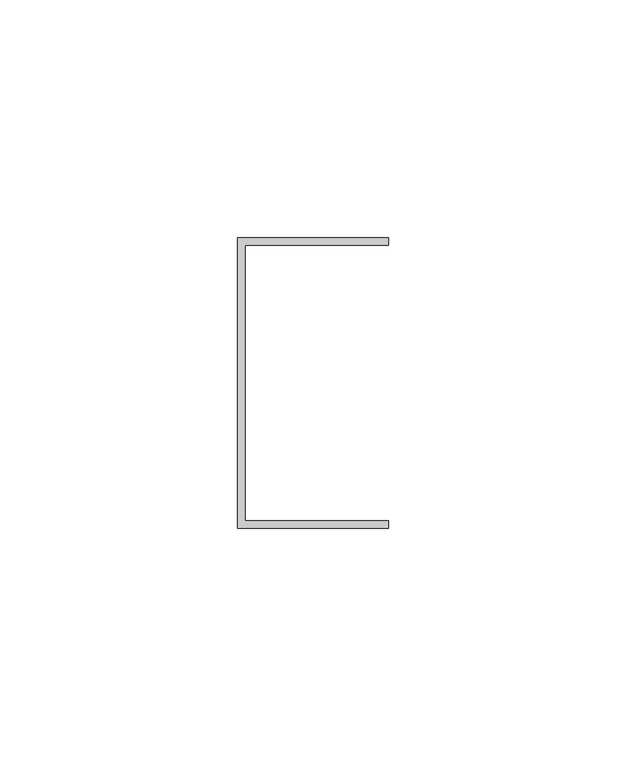
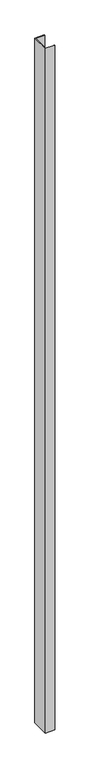
"""IFC4 building model written with IfcOpenShell, lengths in millimetres: proxy geometry, Generic Models 7:Generic Models 1:3:Generic Models 1:3 : Generic Models 7:Generic Models 1:305549:3:Generic Models 1:3:Generic Models 1:3 : Generic Models 7:Generic Models 1:305549:3 : Generic Models 7:Generic Models 1:3:Generic Models 1:3 : Generic Models 7:Generic Models 1:305549:301244:33 : Generic Models 7:Generic Models 1:3:Generic Models 1:3 : Generic Models 7:Generic Models 1:305549:3:Generic Models 1:3:Generic Models 1:3 : Generic Models 7:Generic Models 1:305549:3 : Generic Models 7:Generic Models 1:3:Generic Models 1:3 : Generic Models 7:Generic Models 1:305549:301244:308848."""

import ifcopenshell
import ifcopenshell.guid

model = None  # the IFC model being written
_history = None  # IfcOwnerHistory: only IFC2X3 demands one
_inside = {}  # id of a spatial element -> (the spatial element, [elements in it])
_under = {}  # id of a project, library or spatial element -> (it, [spatial elements below it])
_declared = {}  # id of a project -> (the project, [libraries it declares])
_typed = {}  # id of a type object -> (the type object, [elements of that type])
_made_of = {}  # id of a material, layer set ... -> (it, [elements and type objects made of it])


def new_model(schema):
    """Start an empty IFC model of exactly this schema.

    Asked for "IFC4X3", IfcOpenShell would pick the latest addendum, in which some entities
    have other attributes; the version numbers below select the first issue.
    IFC2X3 requires an IfcOwnerHistory on every rooted entity: one is made here for all.
    """
    global model, _history
    if schema == "IFC4X3":
        model = ifcopenshell.file(schema_version=(4, 3, 0, 0))
    else:
        model = ifcopenshell.file(schema=schema)
    _inside.clear()
    _under.clear()
    _declared.clear()
    _typed.clear()
    _made_of.clear()
    _history = None
    if model.schema == "IFC2X3":
        org = make("IfcOrganization", Name="unknown")
        user = make(
            "IfcPersonAndOrganization",
            ThePerson=make("IfcPerson", FamilyName="unknown"),
            TheOrganization=org,
        )
        app = make(
            "IfcApplication",
            ApplicationDeveloper=org,
            Version="unknown",
            ApplicationFullName="unknown",
            ApplicationIdentifier="unknown",
        )
        _history = make(
            "IfcOwnerHistory",
            OwningUser=user,
            OwningApplication=app,
            ChangeAction="ADDED",
            CreationDate=0,
        )
    return model


def make(cls, **values):
    """One entity of the class cls with the attributes given. An attribute that is None is left unset."""
    return model.create_entity(
        cls, **{name: value for name, value in values.items() if value is not None}
    )


def rooted(cls, **values):
    """An entity with a GlobalId (a new one), such as an element, a storey or a relation."""
    return make(cls, GlobalId=ifcopenshell.guid.new(), OwnerHistory=_history, **values)


def si_unit(unit_type, name, prefix=None):
    """IfcSIUnit, for example si_unit("LENGTHUNIT", "METRE", prefix="MILLI")."""
    return make("IfcSIUnit", UnitType=unit_type, Prefix=prefix, Name=name)


def assignment(units):
    """IfcUnitAssignment: the units of a project."""
    return None if units is None else make("IfcUnitAssignment", Units=units)


def point(xyz):
    """IfcCartesianPoint."""
    return None if xyz is None else make("IfcCartesianPoint", Coordinates=xyz)


def direction(xyz):
    """IfcDirection."""
    return None if xyz is None else make("IfcDirection", DirectionRatios=xyz)


def frame(location, z_axis=None, x_axis=None):
    """IfcAxis2Placement3D, a coordinate frame: its origin and axes. An axis left out is left unset."""
    return make(
        "IfcAxis2Placement3D",
        Location=point(location),
        Axis=direction(z_axis),
        RefDirection=direction(x_axis),
    )


def origin():
    """The frame at (0, 0, 0) with its axes left unset."""
    return frame((0.0, 0.0, 0.0))


def place(relative_to, where):
    """IfcLocalPlacement: puts the frame where relative to a parent placement (None: the world)."""
    return make(
        "IfcLocalPlacement", PlacementRelTo=relative_to, RelativePlacement=where
    )


def context(
    kind, dimensions, precision=None, world=None, true_north=None, identifier=None
):
    """IfcGeometricRepresentationContext, for example the 3D "Model" context."""
    return make(
        "IfcGeometricRepresentationContext",
        ContextIdentifier=identifier,
        ContextType=kind,
        CoordinateSpaceDimension=dimensions,
        Precision=precision,
        WorldCoordinateSystem=world,
        TrueNorth=true_north,
    )


def project(units=None, contexts=None):
    """IfcProject with its units and contexts."""
    return rooted(
        "IfcProject",
        Name="project",
        RepresentationContexts=contexts,
        UnitsInContext=assignment(units),
    )


def spatial(cls, under=None, at=None, **own):
    """A site, building, storey or space (cls), placed at a placement, below another one or the project."""
    s = rooted(cls, ObjectPlacement=at, **own)
    if under is not None:
        _under.setdefault(under.id(), (under, []))[1].append(s)
    return s


def polyline(points):
    """IfcPolyline through the points."""
    return make("IfcPolyline", Points=[point(p) for p in points])


def outline(outer, holes=None, kind="AREA"):
    """IfcArbitraryClosedProfileDef: a profile drawn as a closed curve; with holes, ...WithVoids."""
    if holes is None:
        return make("IfcArbitraryClosedProfileDef", ProfileType=kind, OuterCurve=outer)
    return make(
        "IfcArbitraryProfileDefWithVoids",
        ProfileType=kind,
        OuterCurve=outer,
        InnerCurves=holes,
    )


def extrude(swept, where, along, depth):
    """IfcExtrudedAreaSolid: the profile swept, set in the frame where, extruded along a direction by depth."""
    return make(
        "IfcExtrudedAreaSolid",
        SweptArea=swept,
        Position=where,
        ExtrudedDirection=direction(along),
        Depth=depth,
    )


def shape(context_of_items, identifier, shape_type, items):
    """IfcShapeRepresentation: the items that make up one representation, for example the "Body"."""
    return make(
        "IfcShapeRepresentation",
        ContextOfItems=context_of_items,
        RepresentationIdentifier=identifier,
        RepresentationType=shape_type,
        Items=items,
    )


def source(mapping_origin, context_of_items, identifier, shape_type, items):
    """IfcRepresentationMap: a shape defined once, which mapped items show again and again."""
    return make(
        "IfcRepresentationMap",
        MappingOrigin=mapping_origin,
        MappedRepresentation=shape(context_of_items, identifier, shape_type, items),
    )


def transform(
    local_origin,
    x_axis=None,
    y_axis=None,
    z_axis=None,
    scale=None,
    scale2=None,
    scale3=None,
    uniform=True,
):
    """IfcCartesianTransformationOperator3D, or its non-uniform kind. x_axis, y_axis, z_axis: its Axis1, 2, 3."""
    if uniform:
        return make(
            "IfcCartesianTransformationOperator3D",
            Axis1=direction(x_axis),
            Axis2=direction(y_axis),
            LocalOrigin=point(local_origin),
            Scale=scale,
            Axis3=direction(z_axis),
        )
    return make(
        "IfcCartesianTransformationOperator3DnonUniform",
        Axis1=direction(x_axis),
        Axis2=direction(y_axis),
        LocalOrigin=point(local_origin),
        Scale=scale,
        Axis3=direction(z_axis),
        Scale2=scale2,
        Scale3=scale3,
    )


def mapped(mapping_source, mapping_target):
    """IfcMappedItem: shows the shape of a source again, moved by a transform."""
    return make(
        "IfcMappedItem", MappingSource=mapping_source, MappingTarget=mapping_target
    )


def made_of(thing, what):
    """Note that an element or type object is made of a material, layer set ...; save() writes the relation."""
    if what is not None:
        _made_of.setdefault(what.id(), (what, []))[1].append(thing)
    return thing


def element(
    cls,
    number,
    at=None,
    inside=None,
    cuts=None,
    type_object=None,
    material=None,
    context=None,
    identifier="Body",
    shape_type=None,
    held_by="IfcProductDefinitionShape",
    body=None,
    shapes=None,
    **own,
):
    """One element of the class cls, such as IfcWall. Its Tag is "e" and its number.

    at: its placement. inside: the storey or other place that contains it. cuts: it is an
    opening in that element (IfcRelVoidsElement). A single representation is given by context,
    identifier, shape_type and body (its items); several are given by shapes. held_by: the class
    of the entity that holds the representations. save() writes the other relations.
    """
    e = rooted(cls, Tag="e%d" % number, ObjectPlacement=at, **own)
    if body is not None:
        shapes = [shape(context, identifier, shape_type, body)]
    if shapes is not None:
        e.Representation = make(held_by, Representations=shapes)
    if inside is not None:
        _inside.setdefault(inside.id(), (inside, []))[1].append(e)
    if cuts is not None:
        rooted(
            "IfcRelVoidsElement", RelatingBuildingElement=cuts, RelatedOpeningElement=e
        )
    if type_object is not None:
        _typed.setdefault(type_object.id(), (type_object, []))[1].append(e)
    return made_of(e, material)


def aggregate(whole, parts):
    """IfcRelAggregates: a whole, such as a stair, and the parts it consists of."""
    return rooted("IfcRelAggregates", RelatingObject=whole, RelatedObjects=parts)


def save(model, path):
    """Write the relations noted so far, then the file.

    IfcRelAggregates (storeys below a building ...), IfcRelContainedInSpatialStructure (elements
    in a storey), IfcRelDefinesByType, IfcRelAssociatesMaterial and IfcRelDeclares: one each for
    every whole, place, type object, material and project.
    """
    for whole, parts in _under.values():
        aggregate(whole, parts)
    for where, things in _inside.values():
        rooted(
            "IfcRelContainedInSpatialStructure",
            RelatedElements=things,
            RelatingStructure=where,
        )
    for kind, things in _typed.values():
        rooted("IfcRelDefinesByType", RelatedObjects=things, RelatingType=kind)
    for what, things in _made_of.values():
        rooted("IfcRelAssociatesMaterial", RelatedObjects=things, RelatingMaterial=what)
    for by, libraries in _declared.values():
        rooted("IfcRelDeclares", RelatingContext=by, RelatedDefinitions=libraries)
    model.write(path)


def generic_models_76ce6ccf(model_context):
    return source(origin(), model_context, "Body", "SweptSolid", [
        extrude(outline(polyline([(593757.1367239, -579015.772634), (593788.8867239, -579015.772634), (593788.8867239, -579017.360134), (593758.7242239, -579017.360134), (593758.7242239, -579075.303884), (593788.8867239, -579075.303884), (593788.8867239, -579076.891384), (593757.1367239, -579076.891384), (593757.1367239, -579015.772634)])), frame((0.0, 0.0, 50.8), z_axis=(0.0, 0.0, 1.0), x_axis=(1.0, 0.0, 0.0)), (0.0, 0.0, 1.0), 2430.9324376),
    ])


if __name__ == "__main__":
    model = new_model("IFC4")
    model_context = context("Model", 3, world=origin())
    ifc_project = project(units=[si_unit("LENGTHUNIT", "METRE", prefix="MILLI")], contexts=[model_context])
    site = spatial("IfcSite", under=ifc_project)
    building = spatial("IfcBuilding", under=site)
    placement = place(None, origin())
    generic_models_shape = generic_models_76ce6ccf(model_context)
    element("IfcBuildingElementProxy", 1, Name="Generic Models 7:Generic Models 1:3:Generic Models 1:3 : Generic Models 7:Generic Models 1:305549:3:Generic Models 1:3:Generic Models 1:3 : Generic Models 7:Generic Models 1:305549:3 : Generic Models 7:Generic Models 1:3:Generic Models 1:3 : Generic Models 7:Generic Models 1:305549:301244:33 : Generic Models 7:Generic Models 1:3:Generic Models 1:3 : Generic Models 7:Generic Models 1:305549:3:Generic Models 1:3:Generic Models 1:3 : Generic Models 7:Generic Models 1:305549:3 : Generic Models 7:Generic Models 1:3:Generic Models 1:3 : Generic Models 7:Generic Models 1:305549:301244:308848", ObjectType="Generic Models 7:Generic Models 1:3:Generic Models 1:3 : Generic Models 7:Generic Models 1:305549:3:Generic Models 1:3:Generic Models 1:3 : Generic Models 7:Generic Models 1:305549:3 : Generic Models 7:Generic Models 1:3:Generic Models 1:3 : Generic Models 7:Generic Models 1:305549:301244:33 : Generic Models 7:Generic Models 1:3:Generic Models 1:3 : Generic Models 7:Generic Models 1:305549:3:Generic Models 1:3:Generic Models 1:3 : Generic Models 7:Generic Models 1:305549:3 : Generic Models 7:Generic Models 1:3:Generic Models 1:3 : Generic Models 7:Generic Models 1:305549:301244:308848", at=placement, inside=building, context=model_context, shape_type="MappedRepresentation", body=[
        mapped(generic_models_shape, transform((0.0, 0.0, 0.0), x_axis=(1.0, 0.0, 0.0), y_axis=(0.0, 1.0, 0.0), z_axis=(0.0, 0.0, 1.0))),
    ])
    save(model, "model.ifc")

# Revit data of these elements
# Type "Generic Models 7:Generic Models 1:3:Generic Models 1:3 : Generic Models 7:Generic Models 1:305549:3:Generic Models 1:3:Generic Models 1:3 : Generic Models 7:Generic Models 1:305549:3 : Generic Models 7:Generic Models 1:3:Generic Models 1:3 : Generic Models 7:Generic Models 1:305549:301244:33 : Generic Models 7:Generic Models 1:3:Generic Models 1:3 : Generic Models 7:Generic Models 1:305549:3:Generic Models 1:3:Generic Models 1:3 : Generic Models 7:Generic Models 1:305549:3 : Generic Models 7:Generic Models 1:3:Generic Models 1:3 : Generic Models 7:Generic Models 1:305549:301244:308848"
#   NameOverride = "Generic Models 7:Generic Models 1:3:Generic Models 1:3 : Generic Models 7:Generic Models 1:305549:3:Generic Models 1:3:Generic Models 1:3 : Generic Models 7:Generic Models 1:305549:3 : Generic Models 7:Generic Models 1:3:Generic Models 1:3 : Generic Models 7:Generic Models 1:305549:301244:308848"
#   ObjectTypeOverride = "Generic Models 1:3:Generic Models 1:3 : Generic Models 7:Generic Models 1:305549:3 : Generic Models 7:Generic Models 1:3:Generic Models 1:3 : Generic Models 7:Generic Models 1:305549:301244"
#   Reference = "Generic Models 1"
#   Tag = "308848"
# Element 1 (IfcBuildingElementProxy, "Generic Models 7:Generic Models 1:3:Generic Models 1:3 : Generic Models 7:Generic Models 1:305549:3:Generic Models 1:3:Generic Models 1:3 : Generic Models 7:Generic Models 1:305549:3 : Generic Models 7:Generic Models 1:3:Generic Models 1:3 : Generic Models 7:Generic Models 1:305549:301244:33 : Generic Models 7:Generic Models 1:3:Generic Models 1:3 : Generic Models 7:Generic Models 1:305549:3:Generic Models 1:3:Generic Models 1:3 : Generic Models 7:Generic Models 1:305549:3 : Generic Models 7:Generic Models 1:3:Generic Models 1:3 : Generic Models 7:Generic Models 1:305549:301244:308848")
#   Materials on its faces: "GALVANIZED U-CHANNEL (250T125-33)"
# Materials
#   "GALVANIZED U-CHANNEL (250T125-33)": class "Unassigned", colour RGB 202 201 200, transparency 0, Keynote = "M05451300.02", Cost = 0
